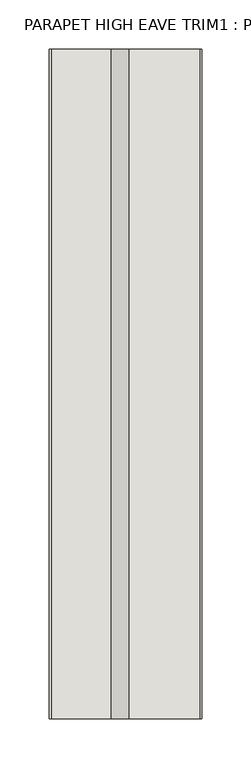
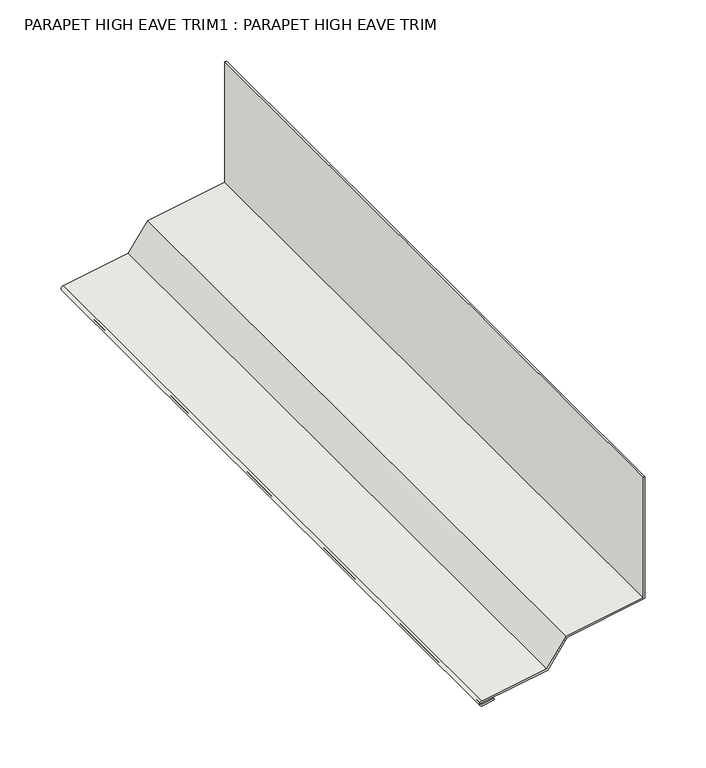
"""IFC4 building model written with IfcOpenShell, lengths in millimetres: wall geometry, PARAPET HIGH EAVE TRIM1 : PARAPET HIGH EAVE TRIM."""

import ifcopenshell
import ifcopenshell.guid

model = None  # the IFC model being written
_history = None  # IfcOwnerHistory: only IFC2X3 demands one
_inside = {}  # id of a spatial element -> (the spatial element, [elements in it])
_under = {}  # id of a project, library or spatial element -> (it, [spatial elements below it])
_declared = {}  # id of a project -> (the project, [libraries it declares])
_typed = {}  # id of a type object -> (the type object, [elements of that type])
_made_of = {}  # id of a material, layer set ... -> (it, [elements and type objects made of it])


def new_model(schema):
    """Start an empty IFC model of exactly this schema.

    Asked for "IFC4X3", IfcOpenShell would pick the latest addendum, in which some entities
    have other attributes; the version numbers below select the first issue.
    IFC2X3 requires an IfcOwnerHistory on every rooted entity: one is made here for all.
    """
    global model, _history
    if schema == "IFC4X3":
        model = ifcopenshell.file(schema_version=(4, 3, 0, 0))
    else:
        model = ifcopenshell.file(schema=schema)
    _inside.clear()
    _under.clear()
    _declared.clear()
    _typed.clear()
    _made_of.clear()
    _history = None
    if model.schema == "IFC2X3":
        org = make("IfcOrganization", Name="unknown")
        user = make(
            "IfcPersonAndOrganization",
            ThePerson=make("IfcPerson", FamilyName="unknown"),
            TheOrganization=org,
        )
        app = make(
            "IfcApplication",
            ApplicationDeveloper=org,
            Version="unknown",
            ApplicationFullName="unknown",
            ApplicationIdentifier="unknown",
        )
        _history = make(
            "IfcOwnerHistory",
            OwningUser=user,
            OwningApplication=app,
            ChangeAction="ADDED",
            CreationDate=0,
        )
    return model


def make(cls, **values):
    """One entity of the class cls with the attributes given. An attribute that is None is left unset."""
    return model.create_entity(
        cls, **{name: value for name, value in values.items() if value is not None}
    )


def rooted(cls, **values):
    """An entity with a GlobalId (a new one), such as an element, a storey or a relation."""
    return make(cls, GlobalId=ifcopenshell.guid.new(), OwnerHistory=_history, **values)


def si_unit(unit_type, name, prefix=None):
    """IfcSIUnit, for example si_unit("LENGTHUNIT", "METRE", prefix="MILLI")."""
    return make("IfcSIUnit", UnitType=unit_type, Prefix=prefix, Name=name)


def assignment(units):
    """IfcUnitAssignment: the units of a project."""
    return None if units is None else make("IfcUnitAssignment", Units=units)


def point(xyz):
    """IfcCartesianPoint."""
    return None if xyz is None else make("IfcCartesianPoint", Coordinates=xyz)


def direction(xyz):
    """IfcDirection."""
    return None if xyz is None else make("IfcDirection", DirectionRatios=xyz)


def frame(location, z_axis=None, x_axis=None):
    """IfcAxis2Placement3D, a coordinate frame: its origin and axes. An axis left out is left unset."""
    return make(
        "IfcAxis2Placement3D",
        Location=point(location),
        Axis=direction(z_axis),
        RefDirection=direction(x_axis),
    )


def frame_2d(location, x_axis=None):
    """IfcAxis2Placement2D, a coordinate frame in the plane: its origin and x axis."""
    return make(
        "IfcAxis2Placement2D", Location=point(location), RefDirection=direction(x_axis)
    )


def origin():
    """The frame at (0, 0, 0) with its axes left unset."""
    return frame((0.0, 0.0, 0.0))


def place(relative_to, where):
    """IfcLocalPlacement: puts the frame where relative to a parent placement (None: the world)."""
    return make(
        "IfcLocalPlacement", PlacementRelTo=relative_to, RelativePlacement=where
    )


def context(
    kind, dimensions, precision=None, world=None, true_north=None, identifier=None
):
    """IfcGeometricRepresentationContext, for example the 3D "Model" context."""
    return make(
        "IfcGeometricRepresentationContext",
        ContextIdentifier=identifier,
        ContextType=kind,
        CoordinateSpaceDimension=dimensions,
        Precision=precision,
        WorldCoordinateSystem=world,
        TrueNorth=true_north,
    )


def project(units=None, contexts=None):
    """IfcProject with its units and contexts."""
    return rooted(
        "IfcProject",
        Name="project",
        RepresentationContexts=contexts,
        UnitsInContext=assignment(units),
    )


def spatial(cls, under=None, at=None, **own):
    """A site, building, storey or space (cls), placed at a placement, below another one or the project."""
    s = rooted(cls, ObjectPlacement=at, **own)
    if under is not None:
        _under.setdefault(under.id(), (under, []))[1].append(s)
    return s


def polyline(points):
    """IfcPolyline through the points."""
    return make("IfcPolyline", Points=[point(p) for p in points])


def circle_curve(where, radius):
    """IfcCircle in the frame where."""
    return make("IfcCircle", Position=where, Radius=radius)


def trimmed(basis, trim1, trim2, sense, master):
    """IfcTrimmedCurve: the piece of a basis curve between two trims."""
    return make(
        "IfcTrimmedCurve",
        BasisCurve=basis,
        Trim1=trim1,
        Trim2=trim2,
        SenseAgreement=sense,
        MasterRepresentation=master,
    )


def segment(curve, same_sense, transition):
    """IfcCompositeCurveSegment."""
    return make(
        "IfcCompositeCurveSegment",
        Transition=transition,
        SameSense=same_sense,
        ParentCurve=curve,
    )


def composite_curve(segments, self_intersect=None):
    """IfcCompositeCurve: segments joined end to end."""
    return make("IfcCompositeCurve", Segments=segments, SelfIntersect=self_intersect)


def outline(outer, holes=None, kind="AREA"):
    """IfcArbitraryClosedProfileDef: a profile drawn as a closed curve; with holes, ...WithVoids."""
    if holes is None:
        return make("IfcArbitraryClosedProfileDef", ProfileType=kind, OuterCurve=outer)
    return make(
        "IfcArbitraryProfileDefWithVoids",
        ProfileType=kind,
        OuterCurve=outer,
        InnerCurves=holes,
    )


def extrude(swept, where, along, depth):
    """IfcExtrudedAreaSolid: the profile swept, set in the frame where, extruded along a direction by depth."""
    return make(
        "IfcExtrudedAreaSolid",
        SweptArea=swept,
        Position=where,
        ExtrudedDirection=direction(along),
        Depth=depth,
    )


def shape(context_of_items, identifier, shape_type, items):
    """IfcShapeRepresentation: the items that make up one representation, for example the "Body"."""
    return make(
        "IfcShapeRepresentation",
        ContextOfItems=context_of_items,
        RepresentationIdentifier=identifier,
        RepresentationType=shape_type,
        Items=items,
    )


def source(mapping_origin, context_of_items, identifier, shape_type, items):
    """IfcRepresentationMap: a shape defined once, which mapped items show again and again."""
    return make(
        "IfcRepresentationMap",
        MappingOrigin=mapping_origin,
        MappedRepresentation=shape(context_of_items, identifier, shape_type, items),
    )


def transform(
    local_origin,
    x_axis=None,
    y_axis=None,
    z_axis=None,
    scale=None,
    scale2=None,
    scale3=None,
    uniform=True,
):
    """IfcCartesianTransformationOperator3D, or its non-uniform kind. x_axis, y_axis, z_axis: its Axis1, 2, 3."""
    if uniform:
        return make(
            "IfcCartesianTransformationOperator3D",
            Axis1=direction(x_axis),
            Axis2=direction(y_axis),
            LocalOrigin=point(local_origin),
            Scale=scale,
            Axis3=direction(z_axis),
        )
    return make(
        "IfcCartesianTransformationOperator3DnonUniform",
        Axis1=direction(x_axis),
        Axis2=direction(y_axis),
        LocalOrigin=point(local_origin),
        Scale=scale,
        Axis3=direction(z_axis),
        Scale2=scale2,
        Scale3=scale3,
    )


def mapped(mapping_source, mapping_target):
    """IfcMappedItem: shows the shape of a source again, moved by a transform."""
    return make(
        "IfcMappedItem", MappingSource=mapping_source, MappingTarget=mapping_target
    )


def made_of(thing, what):
    """Note that an element or type object is made of a material, layer set ...; save() writes the relation."""
    if what is not None:
        _made_of.setdefault(what.id(), (what, []))[1].append(thing)
    return thing


def element(
    cls,
    number,
    at=None,
    inside=None,
    cuts=None,
    type_object=None,
    material=None,
    context=None,
    identifier="Body",
    shape_type=None,
    held_by="IfcProductDefinitionShape",
    body=None,
    shapes=None,
    **own,
):
    """One element of the class cls, such as IfcWall. Its Tag is "e" and its number.

    at: its placement. inside: the storey or other place that contains it. cuts: it is an
    opening in that element (IfcRelVoidsElement). A single representation is given by context,
    identifier, shape_type and body (its items); several are given by shapes. held_by: the class
    of the entity that holds the representations. save() writes the other relations.
    """
    e = rooted(cls, Tag="e%d" % number, ObjectPlacement=at, **own)
    if body is not None:
        shapes = [shape(context, identifier, shape_type, body)]
    if shapes is not None:
        e.Representation = make(held_by, Representations=shapes)
    if inside is not None:
        _inside.setdefault(inside.id(), (inside, []))[1].append(e)
    if cuts is not None:
        rooted(
            "IfcRelVoidsElement", RelatingBuildingElement=cuts, RelatedOpeningElement=e
        )
    if type_object is not None:
        _typed.setdefault(type_object.id(), (type_object, []))[1].append(e)
    return made_of(e, material)


def aggregate(whole, parts):
    """IfcRelAggregates: a whole, such as a stair, and the parts it consists of."""
    return rooted("IfcRelAggregates", RelatingObject=whole, RelatedObjects=parts)


def save(model, path):
    """Write the relations noted so far, then the file.

    IfcRelAggregates (storeys below a building ...), IfcRelContainedInSpatialStructure (elements
    in a storey), IfcRelDefinesByType, IfcRelAssociatesMaterial and IfcRelDeclares: one each for
    every whole, place, type object, material and project.
    """
    for whole, parts in _under.values():
        aggregate(whole, parts)
    for where, things in _inside.values():
        rooted(
            "IfcRelContainedInSpatialStructure",
            RelatedElements=things,
            RelatingStructure=where,
        )
    for kind, things in _typed.values():
        rooted("IfcRelDefinesByType", RelatedObjects=things, RelatingType=kind)
    for what, things in _made_of.values():
        rooted("IfcRelAssociatesMaterial", RelatedObjects=things, RelatingMaterial=what)
    for by, libraries in _declared.values():
        rooted("IfcRelDeclares", RelatingContext=by, RelatedDefinitions=libraries)
    model.write(path)


def parapet_high_eave_trim1_parapet_high_eave_trim_3c361e0f(model_context):
    return source(origin(), model_context, "Body", "SweptSolid", [
        extrude(outline(composite_curve([segment(trimmed(circle_curve(frame_2d((2969.900669, 19440.8352873)), 2.4601541), [point((2972.3234479, 19440.408086))], [point((2967.4778901, 19441.2624886))], False, "CARTESIAN"), True, "CONTINUOUS"), segment(polyline([(2967.4778901, 19441.2624886), (2969.3880604, 19452.0956023), (2970.9514427, 19451.8199358), (2969.0412725, 19440.9868221)]), True, "CONTINUOUS"), segment(trimmed(circle_curve(frame_2d((2969.8229636, 19440.8489888)), 0.79375), [point((2969.0412725, 19440.9868221))], [point((2970.6046548, 19440.7111556))], True, "CARTESIAN"), True, "CONTINUOUS"), segment(polyline([(2970.6046548, 19440.7111556), (2981.4984378, 19502.4928692), (3007.8543253, 19520.9474603), (3020.7559715, 19594.1163317), (3142.0720068, 19594.1163317), (3142.0720068, 19592.5288317), (3022.0880421, 19592.5288317), (3009.3035228, 19520.0242196), (2983.1304492, 19501.6976362), (2972.3234479, 19440.408086)]), True, "CONTINUOUS")], self_intersect=False)), frame((0.0, -2319.6634634, 0.0), z_axis=(0.0, 1.0, 0.0), x_axis=(0.0, 0.0, 1.0)), (0.0, 0.0, 1.0), 682.625),
    ])


if __name__ == "__main__":
    model = new_model("IFC4")
    model_context = context("Model", 3, world=origin())
    ifc_project = project(units=[si_unit("LENGTHUNIT", "METRE", prefix="MILLI")], contexts=[model_context])
    site = spatial("IfcSite", under=ifc_project)
    building = spatial("IfcBuilding", under=site)
    placement = place(None, origin())
    parapet_high_eave_trim1_parapet_high_eave_trim_shape = parapet_high_eave_trim1_parapet_high_eave_trim_3c361e0f(model_context)
    element("IfcWall", 1, ObjectType="PARAPET HIGH EAVE TRIM1 : PARAPET HIGH EAVE TRIM", at=placement, inside=building, context=model_context, shape_type="MappedRepresentation", body=[
        mapped(parapet_high_eave_trim1_parapet_high_eave_trim_shape, transform((0.0, 0.0, 0.0), x_axis=(1.0, 0.0, 0.0), y_axis=(0.0, 1.0, 0.0), z_axis=(0.0, 0.0, 1.0))),
    ])
    save(model, "model.ifc")

# Revit data of these elements
# Element 1 (IfcWall, "PARAPET HIGH EAVE TRIM1 : PARAPET HIGH EAVE TRIM")
#   Materials on its faces: "PARAPET HIGH EAVE TRIM"
# Materials
#   "PARAPET HIGH EAVE TRIM": class "Metal", colour RGB 247 247 247, transparency 0, Cost = 0
